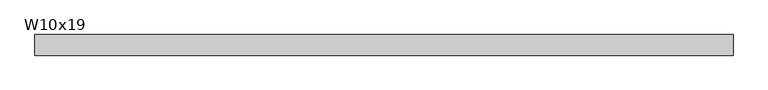
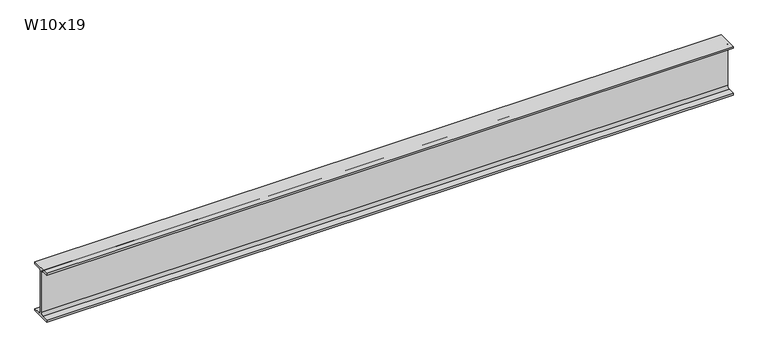
"""IFC4 building model written with IfcOpenShell, lengths in millimetres: beam geometry, RME W-Wide Flange : W10x19."""

from ifc_helpers import new_model, si_unit, point, frame, frame_2d, origin, place, context, project, spatial, polyline, circle_curve, trimmed, segment, composite_curve, outline, extrude, source, transform, mapped, element, save


def w10x19_80c7dafd(model_context):
    return source(origin(), model_context, "Body", "SweptSolid", [
        extrude(outline(composite_curve([segment(polyline([(51.054, -119.507), (51.054, -129.54), (-51.054, -129.54), (-51.054, -119.507), (-16.9545, -119.507)]), True, "CONTINUOUS"), segment(trimmed(circle_curve(frame_2d((-16.9545, -105.7275)), 13.7795), [point((-16.9545, -119.507))], [point((-3.175, -105.7275))], True, "CARTESIAN"), True, "CONTINUOUS"), segment(polyline([(-3.175, -105.7275), (-3.175, 105.7275)]), True, "CONTINUOUS"), segment(trimmed(circle_curve(frame_2d((-16.9545, 105.7275)), 13.7795), [point((-3.175, 105.7275))], [point((-16.9545, 119.507))], True, "CARTESIAN"), True, "CONTINUOUS"), segment(polyline([(-16.9545, 119.507), (-51.054, 119.507), (-51.054, 129.54), (51.054, 129.54), (51.054, 119.507), (16.9545, 119.507)]), True, "CONTINUOUS"), segment(trimmed(circle_curve(frame_2d((16.9545, 105.7275)), 13.7795), [point((16.9545, 119.507))], [point((3.175, 105.7275))], True, "CARTESIAN"), True, "CONTINUOUS"), segment(polyline([(3.175, 105.7275), (3.175, -105.7275)]), True, "CONTINUOUS"), segment(trimmed(circle_curve(frame_2d((16.9545, -105.7275)), 13.7795), [point((3.175, -105.7275))], [point((16.9545, -119.507))], True, "CARTESIAN"), True, "CONTINUOUS"), segment(polyline([(16.9545, -119.507), (51.054, -119.507)]), True, "CONTINUOUS")], self_intersect=False)), frame((-1732.5793379, 0.0, 0.0), z_axis=(1.0, 0.0, 0.0), x_axis=(0.0, 1.0, 0.0)), (0.0, 0.0, 1.0), 3457.6885493),
    ])


if __name__ == "__main__":
    model = new_model("IFC4")
    model_context = context("Model", 3, world=origin())
    ifc_project = project(units=[si_unit("LENGTHUNIT", "METRE", prefix="MILLI")], contexts=[model_context])
    site = spatial("IfcSite", under=ifc_project)
    building = spatial("IfcBuilding", under=site)
    placement = place(None, origin())
    w10x19_shape = w10x19_80c7dafd(model_context)
    element("IfcBeam", 1, ObjectType="RME W-Wide Flange : W10x19", at=placement, inside=building, context=model_context, shape_type="MappedRepresentation", body=[
        mapped(w10x19_shape, transform((0.0, 0.0, 0.0), x_axis=(1.0, 0.0, 0.0), y_axis=(0.0, 1.0, 0.0), z_axis=(0.0, 0.0, 1.0))),
    ])
    save(model, "model.ifc")

# Revit data of these elements
# Type "RME W-Wide Flange : W10x19"
#   WELD P [instance default] = ""
#   WELD LE [instance default] = ""
#   WELD D [instance default] = ""
#   TOP SECTION SIZE [instance default] = ""
#   TOP SECTION LENGTH [instance default] = ""
#   REMARKS [instance default] = ""
#   REINF TYPE [instance default] = ""
#   Nominal Size = "W24"
#   End Bearing Capacity [instance default] = ""
#   BOT SECTION SIZE [instance default] = ""
#   BOT SECTION LENGTH [instance default] = ""
#   Assembly Code = "B10"
#   W = 19
#   Start Extension Calculation [instance default] = 10' - 0"
#   Start Extension [instance default] = -0' - 0 1/2"
#   End Extension Calculation [instance default] = 10' - 0"
#   End Extension [instance default] = -0' - 0 1/2"
#   Length [instance default] = 5' - 0"
#   bf = 0' - 4.02"
#   d = 0' - 10.2"
#   k = 0' - 0 15/16"
#   k2 = 0' - 0.5425"
#   tf = 0' - 0.395"
#   tw = 0' - 0 1/4"
#   A = 0.0390278 SF
#   Structural Material [instance default] = Metal - Steel - ASTM A992
# Element 1 (IfcBeam, "RME W-Wide Flange : W10x19")
#   Length = 11' - 10.86522"
#   Materials on its faces: "Metal - Steel - ASTM A992"
# Materials
#   "Metal - Steel - ASTM A992": class "Metal", colour RGB 255 128 0, transparency 0
